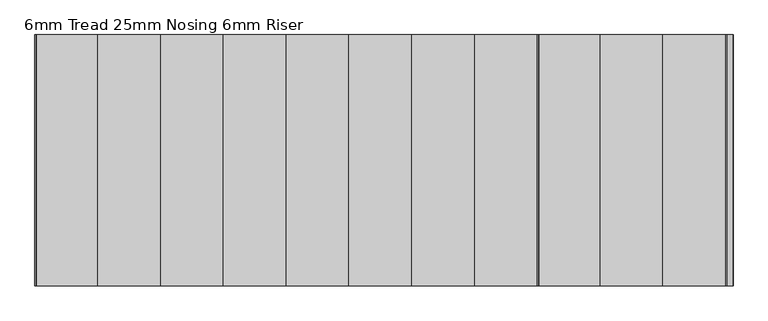
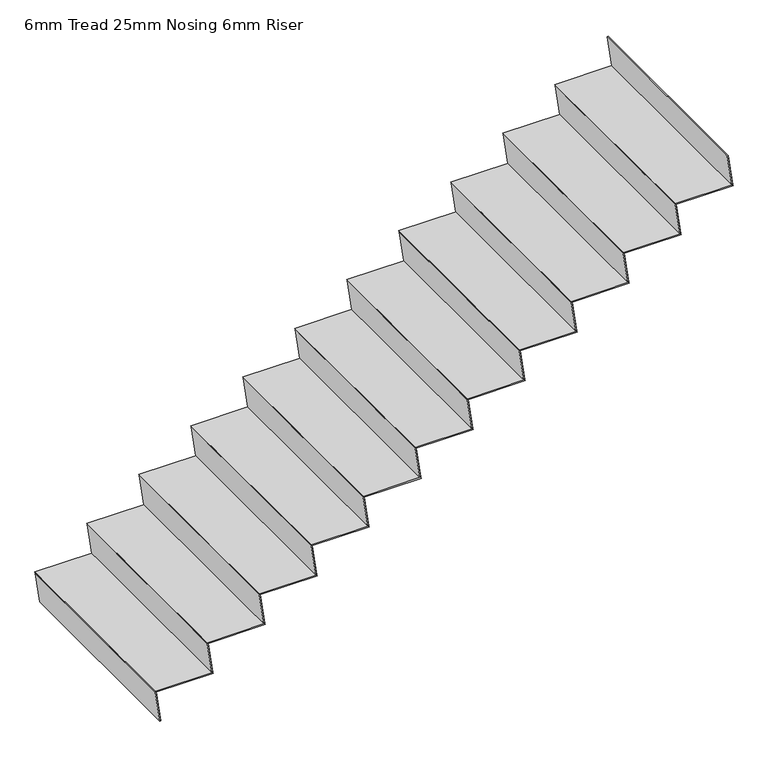
"""IFC4 building model written with IfcOpenShell, lengths in millimetres: stair flight geometry, 6mm Tread 25mm Nosing 6mm Riser."""

from ifc_helpers import new_model, si_unit, frame, origin, place, context, project, spatial, polyline, outline, extrude, source, transform, mapped, element, save


def stair_flight_6mm_tread_25mm_nosing_6mm_riser_1db906a5(model_context):
    return source(origin(), model_context, "Body", "SweptSolid", [
        extrude(outline(polyline([(24411.7647059, 13631.0599092), (24411.7647059, 13325.0), (24405.7647059, 13325.85), (24405.7647059, 13631.9099092), (24411.7647059, 13631.0599092)])), frame((0.0, 10295.4345331, 0.0), z_axis=(0.0, 1.0, 0.0), x_axis=(0.0, 0.0, 1.0)), (0.0, 0.0, 1.0), 1100.0),
        extrude(outline(polyline([(24405.7647059, 13325.85), (24235.2941176, 13350.0), (24235.2941176, 13356.0599092), (24405.7647059, 13331.9099092), (24405.7647059, 13325.85)])), frame((0.0, 10295.4345331, 0.0), z_axis=(0.0, 1.0, 0.0), x_axis=(0.0, 0.0, 1.0)), (0.0, 0.0, 1.0), 1100.0),
        extrude(outline(polyline([(24582.2352941, 13600.85), (24411.7647059, 13625.0), (24411.7647059, 13631.0599092), (24582.2352941, 13606.9099092), (24582.2352941, 13600.85)])), frame((0.0, 10295.4345331, 0.0), z_axis=(0.0, 1.0, 0.0), x_axis=(0.0, 0.0, 1.0)), (0.0, 0.0, 1.0), 1100.0),
        extrude(outline(polyline([(24588.2352941, 13906.0599092), (24588.2352941, 13600.0), (24582.2352941, 13600.85), (24582.2352941, 13906.9099092), (24588.2352941, 13906.0599092)])), frame((0.0, 10295.4345331, 0.0), z_axis=(0.0, 1.0, 0.0), x_axis=(0.0, 0.0, 1.0)), (0.0, 0.0, 1.0), 1100.0),
        extrude(outline(polyline([(24758.7058824, 13875.85), (24588.2352941, 13900.0), (24588.2352941, 13906.0599092), (24758.7058824, 13881.9099092), (24758.7058824, 13875.85)])), frame((0.0, 10295.4345331, 0.0), z_axis=(0.0, 1.0, 0.0), x_axis=(0.0, 0.0, 1.0)), (0.0, 0.0, 1.0), 1100.0),
        extrude(outline(polyline([(24764.7058824, 14181.0599092), (24764.7058824, 13875.0), (24758.7058824, 13875.85), (24758.7058824, 14181.9099092), (24764.7058824, 14181.0599092)])), frame((0.0, 10295.4345331, 0.0), z_axis=(0.0, 1.0, 0.0), x_axis=(0.0, 0.0, 1.0)), (0.0, 0.0, 1.0), 1100.0),
        extrude(outline(polyline([(24935.1764706, 14150.85), (24764.7058824, 14175.0), (24764.7058824, 14181.0599092), (24935.1764706, 14156.9099092), (24935.1764706, 14150.85)])), frame((0.0, 10295.4345331, 0.0), z_axis=(0.0, 1.0, 0.0), x_axis=(0.0, 0.0, 1.0)), (0.0, 0.0, 1.0), 1100.0),
        extrude(outline(polyline([(24941.1764706, 14456.0599092), (24941.1764706, 14150.0), (24935.1764706, 14150.85), (24935.1764706, 14456.9099092), (24941.1764706, 14456.0599092)])), frame((0.0, 10295.4345331, 0.0), z_axis=(0.0, 1.0, 0.0), x_axis=(0.0, 0.0, 1.0)), (0.0, 0.0, 1.0), 1100.0),
        extrude(outline(polyline([(25111.6470588, 14425.85), (24941.1764706, 14450.0), (24941.1764706, 14456.0599092), (25111.6470588, 14431.9099092), (25111.6470588, 14425.85)])), frame((0.0, 10295.4345331, 0.0), z_axis=(0.0, 1.0, 0.0), x_axis=(0.0, 0.0, 1.0)), (0.0, 0.0, 1.0), 1100.0),
        extrude(outline(polyline([(25117.6470588, 14731.0599092), (25117.6470588, 14425.0), (25111.6470588, 14425.85), (25111.6470588, 14731.9099092), (25117.6470588, 14731.0599092)])), frame((0.0, 10295.4345331, 0.0), z_axis=(0.0, 1.0, 0.0), x_axis=(0.0, 0.0, 1.0)), (0.0, 0.0, 1.0), 1100.0),
        extrude(outline(polyline([(25288.1176471, 14700.85), (25117.6470588, 14725.0), (25117.6470588, 14731.0599092), (25288.1176471, 14706.9099092), (25288.1176471, 14700.85)])), frame((0.0, 10295.4345331, 0.0), z_axis=(0.0, 1.0, 0.0), x_axis=(0.0, 0.0, 1.0)), (0.0, 0.0, 1.0), 1100.0),
        extrude(outline(polyline([(25294.1176471, 15006.0599092), (25294.1176471, 14700.0), (25288.1176471, 14700.85), (25288.1176471, 15006.9099092), (25294.1176471, 15006.0599092)])), frame((0.0, 10295.4345331, 0.0), z_axis=(0.0, 1.0, 0.0), x_axis=(0.0, 0.0, 1.0)), (0.0, 0.0, 1.0), 1100.0),
        extrude(outline(polyline([(25464.5882353, 14975.85), (25294.1176471, 15000.0), (25294.1176471, 15006.0599092), (25464.5882353, 14981.9099092), (25464.5882353, 14975.85)])), frame((0.0, 10295.4345331, 0.0), z_axis=(0.0, 1.0, 0.0), x_axis=(0.0, 0.0, 1.0)), (0.0, 0.0, 1.0), 1100.0),
        extrude(outline(polyline([(25470.5882353, 15281.0599092), (25470.5882353, 14975.0), (25464.5882353, 14975.85), (25464.5882353, 15281.9099092), (25470.5882353, 15281.0599092)])), frame((0.0, 10295.4345331, 0.0), z_axis=(0.0, 1.0, 0.0), x_axis=(0.0, 0.0, 1.0)), (0.0, 0.0, 1.0), 1100.0),
        extrude(outline(polyline([(25641.0588235, 15250.85), (25470.5882353, 15275.0), (25470.5882353, 15281.0599092), (25641.0588235, 15256.9099092), (25641.0588235, 15250.85)])), frame((0.0, 10295.4345331, 0.0), z_axis=(0.0, 1.0, 0.0), x_axis=(0.0, 0.0, 1.0)), (0.0, 0.0, 1.0), 1100.0),
        extrude(outline(polyline([(25647.0588235, 15556.0599092), (25647.0588235, 15250.0), (25641.0588235, 15250.85), (25641.0588235, 15556.9099092), (25647.0588235, 15556.0599092)])), frame((0.0, 10295.4345331, 0.0), z_axis=(0.0, 1.0, 0.0), x_axis=(0.0, 0.0, 1.0)), (0.0, 0.0, 1.0), 1100.0),
        extrude(outline(polyline([(25817.5294118, 15525.85), (25647.0588235, 15550.0), (25647.0588235, 15556.0599092), (25817.5294118, 15531.9099092), (25817.5294118, 15525.85)])), frame((0.0, 10295.4345331, 0.0), z_axis=(0.0, 1.0, 0.0), x_axis=(0.0, 0.0, 1.0)), (0.0, 0.0, 1.0), 1100.0),
        extrude(outline(polyline([(25823.5294118, 15831.0599092), (25823.5294118, 15525.0), (25817.5294118, 15525.85), (25817.5294118, 15831.9099092), (25823.5294118, 15831.0599092)])), frame((0.0, 10295.4345331, 0.0), z_axis=(0.0, 1.0, 0.0), x_axis=(0.0, 0.0, 1.0)), (0.0, 0.0, 1.0), 1100.0),
        extrude(outline(polyline([(25994.0, 15800.85), (25823.5294118, 15825.0), (25823.5294118, 15831.0599092), (25994.0, 15806.9099092), (25994.0, 15800.85)])), frame((0.0, 10295.4345331, 0.0), z_axis=(0.0, 1.0, 0.0), x_axis=(0.0, 0.0, 1.0)), (0.0, 0.0, 1.0), 1100.0),
        extrude(outline(polyline([(26000.0, 16106.0599092), (26000.0, 15800.0), (25994.0, 15800.85), (25994.0, 16106.9099092), (26000.0, 16106.0599092)])), frame((0.0, 10295.4345331, 0.0), z_axis=(0.0, 1.0, 0.0), x_axis=(0.0, 0.0, 1.0)), (0.0, 0.0, 1.0), 1100.0),
        extrude(outline(polyline([(26170.4705882, 16075.85), (26000.0, 16100.0), (26000.0, 16106.0599092), (26170.4705882, 16081.9099092), (26170.4705882, 16075.85)])), frame((0.0, 10295.4345331, 0.0), z_axis=(0.0, 1.0, 0.0), x_axis=(0.0, 0.0, 1.0)), (0.0, 0.0, 1.0), 1100.0),
        extrude(outline(polyline([(26346.9411765, 16350.85), (26176.4705882, 16375.0), (26176.4705882, 16381.0599092), (26346.9411765, 16356.9099092), (26346.9411765, 16350.85)])), frame((0.0, 10295.4345331, 0.0), z_axis=(0.0, 1.0, 0.0), x_axis=(0.0, 0.0, 1.0)), (0.0, 0.0, 1.0), 1100.0),
        extrude(outline(polyline([(26176.4705882, 16381.0599092), (26176.4705882, 16075.0), (26170.4705882, 16075.85), (26170.4705882, 16381.9099092), (26176.4705882, 16381.0599092)])), frame((0.0, 10295.4345331, 0.0), z_axis=(0.0, 1.0, 0.0), x_axis=(0.0, 0.0, 1.0)), (0.0, 0.0, 1.0), 1100.0),
    ])


if __name__ == "__main__":
    model = new_model("IFC4")
    model_context = context("Model", 3, world=origin())
    ifc_project = project(units=[si_unit("LENGTHUNIT", "METRE", prefix="MILLI")], contexts=[model_context])
    site = spatial("IfcSite", under=ifc_project)
    building = spatial("IfcBuilding", under=site)
    placement = place(None, origin())
    stair_flight_6mm_tread_25mm_nosing_6mm_riser_shape = stair_flight_6mm_tread_25mm_nosing_6mm_riser_1db906a5(model_context)
    element("IfcStairFlight", 1, ObjectType="6mm Tread 25mm Nosing 6mm Riser", at=placement, inside=building, context=model_context, shape_type="MappedRepresentation", body=[
        mapped(stair_flight_6mm_tread_25mm_nosing_6mm_riser_shape, transform((0.0, 0.0, 0.0), x_axis=(1.0, 0.0, 0.0), y_axis=(0.0, 1.0, 0.0), z_axis=(0.0, 0.0, 1.0))),
    ])
    save(model, "model.ifc")

# Revit data of these elements
# Element 1 (IfcStairFlight, "6mm Tread 25mm Nosing 6mm Riser")
#   Materials on its faces: "Steel, Paint Finish, Dark Gray"
# Materials
#   "Steel, Paint Finish, Dark Gray": class "Metal", colour RGB 89 89 89, transparency 0, Description = "Steel, paint finish, dark gray, glossy", Cost = 0
